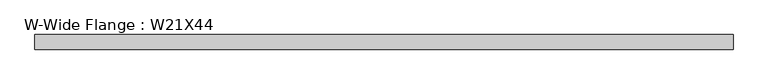
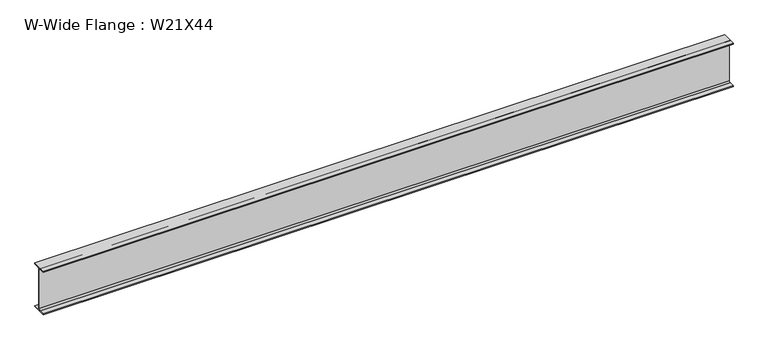
"""IFC4 building model written with IfcOpenShell, lengths in millimetres: beam geometry, W-Wide Flange : W21X44."""

from ifc_helpers import new_model, si_unit, point, frame, frame_2d, origin, place, context, project, spatial, polyline, circle_curve, trimmed, segment, composite_curve, outline, extrude, source, transform, mapped, element, save


def w_wide_flange_w21x44_dd8e647a(model_context):
    return source(origin(), model_context, "Body", "SweptSolid", [
        extrude(outline(composite_curve([segment(polyline([(82.55, -251.46), (82.55, -262.89), (-82.55, -262.89), (-82.55, -251.46), (-21.59, -251.46)]), True, "CONTINUOUS"), segment(trimmed(circle_curve(frame_2d((-21.59, -234.315)), 17.145), [point((-21.59, -251.46))], [point((-4.445, -234.315))], True, "CARTESIAN"), True, "CONTINUOUS"), segment(polyline([(-4.445, -234.315), (-4.445, 234.315)]), True, "CONTINUOUS"), segment(trimmed(circle_curve(frame_2d((-21.59, 234.315)), 17.145), [point((-4.445, 234.315))], [point((-21.59, 251.46))], True, "CARTESIAN"), True, "CONTINUOUS"), segment(polyline([(-21.59, 251.46), (-82.55, 251.46), (-82.55, 262.89), (82.55, 262.89), (82.55, 251.46), (21.59, 251.46)]), True, "CONTINUOUS"), segment(trimmed(circle_curve(frame_2d((21.59, 234.315)), 17.145), [point((21.59, 251.46))], [point((4.445, 234.315))], True, "CARTESIAN"), True, "CONTINUOUS"), segment(polyline([(4.445, 234.315), (4.445, -234.315)]), True, "CONTINUOUS"), segment(trimmed(circle_curve(frame_2d((21.59, -234.315)), 17.145), [point((4.445, -234.315))], [point((21.59, -251.46))], True, "CARTESIAN"), True, "CONTINUOUS"), segment(polyline([(21.59, -251.46), (82.55, -251.46)]), True, "CONTINUOUS")], self_intersect=False)), frame((-3902.8286345, 0.0, 0.0), z_axis=(1.0, 0.0, 0.0), x_axis=(0.0, 1.0, 0.0)), (0.0, 0.0, 1.0), 7866.3605813),
    ])


if __name__ == "__main__":
    model = new_model("IFC4")
    model_context = context("Model", 3, world=origin())
    ifc_project = project(units=[si_unit("LENGTHUNIT", "METRE", prefix="MILLI")], contexts=[model_context])
    site = spatial("IfcSite", under=ifc_project)
    building = spatial("IfcBuilding", under=site)
    placement = place(None, origin())
    w_wide_flange_w21x44_shape = w_wide_flange_w21x44_dd8e647a(model_context)
    element("IfcBeam", 1, ObjectType="W-Wide Flange : W21X44", at=placement, inside=building, context=model_context, shape_type="MappedRepresentation", body=[
        mapped(w_wide_flange_w21x44_shape, transform((0.0, 0.0, 0.0), x_axis=(1.0, 0.0, 0.0), y_axis=(0.0, 1.0, 0.0), z_axis=(0.0, 0.0, 1.0))),
    ])
    save(model, "model.ifc")

# Revit data of these elements
# Type "W-Wide Flange : W21X44"
#   Assembly Code = "B10"
#   W = 44
#   Length [instance default] = 1524 mm
#   bf = 165.1 mm
#   d = 525.78 mm
#   k = 28.575 mm
#   k2 = 17.145 mm
#   tf = 11.43 mm
#   tw = 8.89 mm
#   A = 0.00838708 m²
#   Structural Material [instance default] = Steel ASTM A992
# Element 1 (IfcBeam, "W-Wide Flange : W21X44")
#   Structural Material = Aluminum, Anodized Red
#   Materials on its faces: "Aluminum, Anodized Red"
# Materials
#   "Steel ASTM A992": class "Metal", colour RGB 128 0 0, transparency 0, Description = "Structural steel 50ksi", Cost = 0
#   "Aluminum, Anodized Red": class "Metal", colour RGB 120 120 120, transparency 0, Description = "Anodized aluminum, red", Cost = 0
